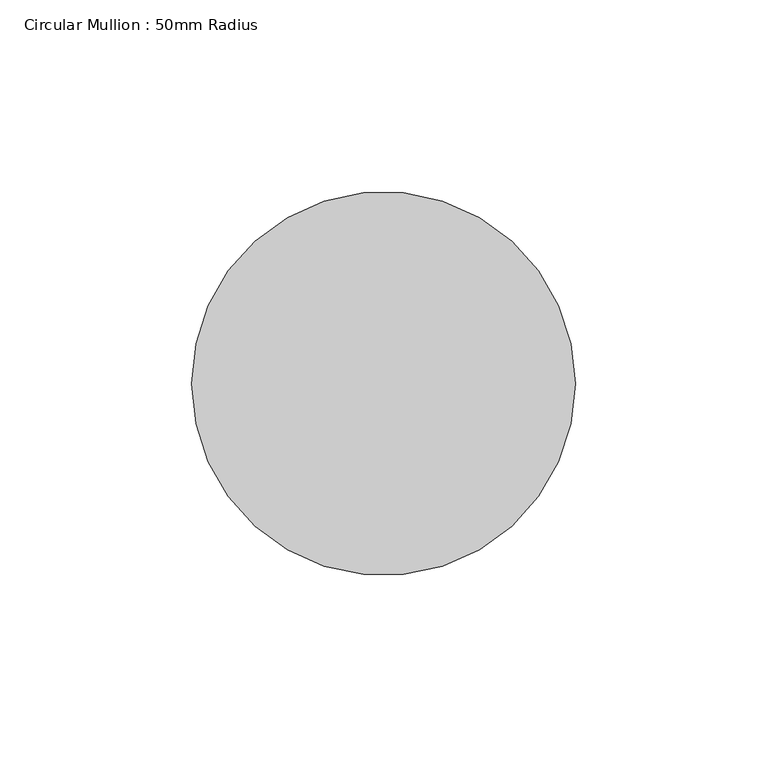
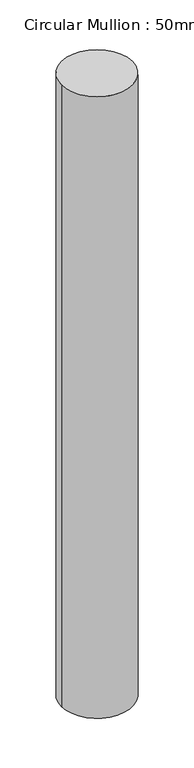
"""IFC4 building model written with IfcOpenShell, lengths in millimetres: member geometry, Circular Mullion : 50mm Radius."""

from ifc_helpers import new_model, si_unit, point, frame, origin, origin_2d, place, context, project, spatial, circle_curve, trimmed, segment, composite_curve, outline, extrude, source, transform, mapped, element, save


def circular_mullion_50mm_radius_51db2a0a(model_context):
    return source(origin(), model_context, "Body", "SweptSolid", [
        extrude(outline(composite_curve([segment(trimmed(circle_curve(origin_2d(), 50.0), [point((50.0, 0.0))], [point((-50.0, 0.0))], False, "CARTESIAN"), True, "CONTINUOUS"), segment(trimmed(circle_curve(origin_2d(), 50.0), [point((-50.0, 0.0))], [point((50.0, 0.0))], False, "CARTESIAN"), True, "CONTINUOUS")], self_intersect=False)), frame((0.0, 0.0, -924.1733061), z_axis=(0.0, 0.0, 1.0), x_axis=(1.0, 0.0, 0.0)), (0.0, 0.0, 1.0), 924.1733061),
    ])


if __name__ == "__main__":
    model = new_model("IFC4")
    model_context = context("Model", 3, world=origin())
    ifc_project = project(units=[si_unit("LENGTHUNIT", "METRE", prefix="MILLI")], contexts=[model_context])
    site = spatial("IfcSite", under=ifc_project)
    building = spatial("IfcBuilding", under=site)
    placement = place(None, origin())
    circular_mullion_50mm_radius_shape = circular_mullion_50mm_radius_51db2a0a(model_context)
    element("IfcMember", 1, ObjectType="Circular Mullion : 50mm Radius", at=placement, inside=building, context=model_context, shape_type="MappedRepresentation", body=[
        mapped(circular_mullion_50mm_radius_shape, transform((0.0, 0.0, 0.0), x_axis=(1.0, 0.0, 0.0), y_axis=(0.0, 1.0, 0.0), z_axis=(0.0, 0.0, 1.0))),
    ])
    save(model, "model.ifc")

# Revit data of these elements
# Type "Circular Mullion : 50mm Radius"
#   built-in parameter 1007350 = 0.164042 (stored number, unit not read)
# Element 1 (IfcMember, "Circular Mullion : 50mm Radius")
#   Materials on its faces: "Aluminium"
# Materials
#   "Aluminium": class "Metal", colour RGB 247 247 247, transparency 0, Description = "Aluminium 6061", Cost = 0
